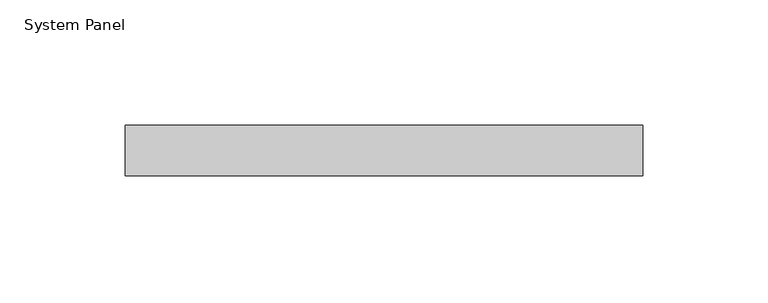
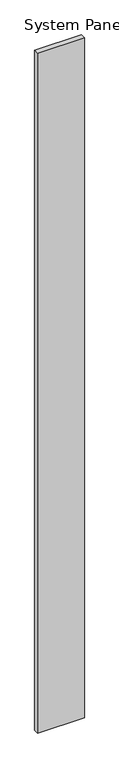
"""IFC4 building model written with IfcOpenShell, lengths in millimetres: plate geometry, System Panel : WWm-Glass-20mm-10mmOffset."""

from ifc_helpers import new_model, si_unit, origin, origin_with_axes, place, context, project, spatial, polyline, outline, extrude, source, transform, mapped, element, save


def system_panel_867956c0(model_context):
    return source(origin(), model_context, "Body", "SweptSolid", [
        extrude(outline(polyline([(102.9990727, 0.0), (-102.9990727, 0.0), (-102.9990727, 20.0), (102.9990727, 20.0), (102.9990727, 0.0)])), origin_with_axes(), (0.0, 0.0, 1.0), 3150.0),
    ])


if __name__ == "__main__":
    model = new_model("IFC4")
    model_context = context("Model", 3, world=origin())
    ifc_project = project(units=[si_unit("LENGTHUNIT", "METRE", prefix="MILLI")], contexts=[model_context])
    site = spatial("IfcSite", under=ifc_project)
    building = spatial("IfcBuilding", under=site)
    placement = place(None, origin())
    system_panel_shape = system_panel_867956c0(model_context)
    element("IfcPlate", 1, ObjectType="System Panel : WWm-Glass-20mm-10mmOffset", at=placement, inside=building, context=model_context, shape_type="MappedRepresentation", body=[
        mapped(system_panel_shape, transform((0.0, 0.0, 0.0), x_axis=(1.0, 0.0, 0.0), y_axis=(0.0, 1.0, 0.0), z_axis=(0.0, 0.0, 1.0))),
    ])
    save(model, "model.ifc")

# Revit data of these elements
# Type "System Panel : WWm-Glass-20mm-10mmOffset"
#   Finish = ""
# Element 1 (IfcPlate, "System Panel : WWm-Glass-20mm-10mmOffset")
#   Materials on its faces: "WW-EC-GL-Storefront"
# Materials
#   "WW-EC-GL-Storefront": class "Glass", colour RGB 236 240 239, transparency 0.85, Description = "Storefront Glass", Cost = 0
